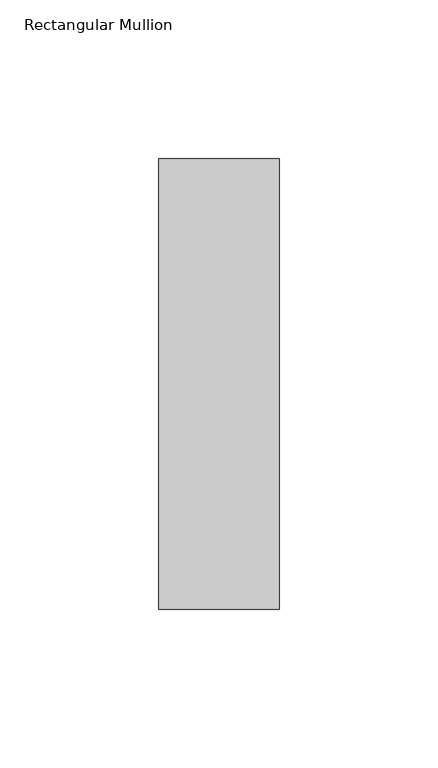
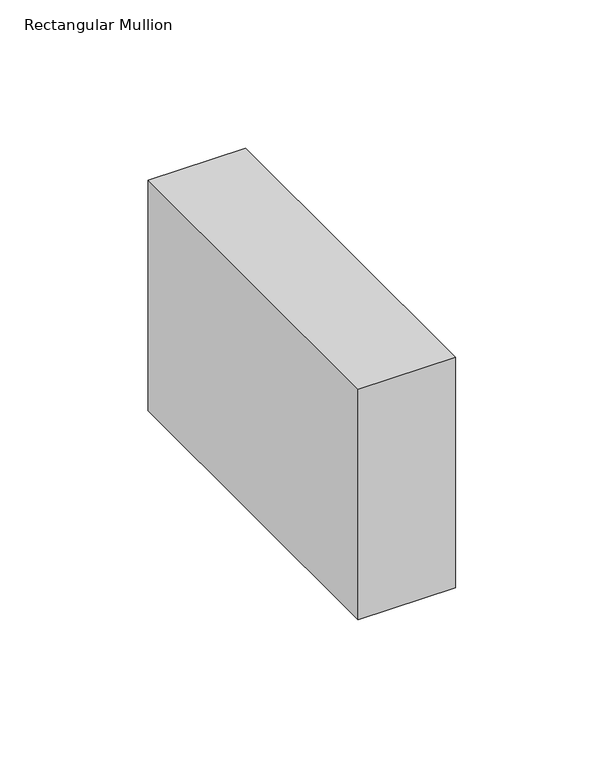
"""IFC4 building model written with IfcOpenShell, lengths in millimetres: member geometry, Rectangular Mullion : NLRS_21_CWM_hsb-regel 38x142_gen_rsf."""

from ifc_helpers import new_model, si_unit, frame, origin, place, context, project, spatial, polyline, outline, extrude, source, transform, mapped, element, save


def rectangular_mullion_3dbdc851(model_context):
    return source(origin(), model_context, "Body", "SweptSolid", [
        extrude(outline(polyline([(-38.0, -71.0), (-38.0, 71.0), (0.0, 71.0), (0.0, -71.0), (-38.0, -71.0)])), frame((0.0, 0.0, -94.9999997), z_axis=(0.0, 0.0, 1.0), x_axis=(1.0, 0.0, 0.0)), (0.0, 0.0, 1.0), 94.9999997),
    ])


if __name__ == "__main__":
    model = new_model("IFC4")
    model_context = context("Model", 3, world=origin())
    ifc_project = project(units=[si_unit("LENGTHUNIT", "METRE", prefix="MILLI")], contexts=[model_context])
    site = spatial("IfcSite", under=ifc_project)
    building = spatial("IfcBuilding", under=site)
    placement = place(None, origin())
    rectangular_mullion_shape = rectangular_mullion_3dbdc851(model_context)
    element("IfcMember", 1, ObjectType="Rectangular Mullion : NLRS_21_CWM_hsb-regel 38x142_gen_rsf", at=placement, inside=building, context=model_context, shape_type="MappedRepresentation", body=[
        mapped(rectangular_mullion_shape, transform((0.0, 0.0, 0.0), x_axis=(1.0, 0.0, 0.0), y_axis=(0.0, 1.0, 0.0), z_axis=(0.0, 0.0, 1.0))),
    ])
    save(model, "model.ifc")

# Revit data of these elements
# Type "Rectangular Mullion : NLRS_21_CWM_hsb-regel 38x142_gen_rsf"
#   Export Type to IFC As = "IfcWall"
#   Type IfcGUID = "07M7mRoiH1CR8m_RSKIwpF"
#   Assembly Code = "21.10"
#   built-in parameter 1007322 = 0.465879 (stored number, unit not read)
#   built-in parameter 1007321 = 0.062336 (stored number, unit not read)
#   built-in parameter 1007320 = 0.062336 (stored number, unit not read)
# Element 1 (IfcMember, "Rectangular Mullion : NLRS_21_CWM_hsb-regel 38x142_gen_rsf")
#   Materials on its faces: "NLRS_i2_hout naaldhout vuren_gen_rsf"
# Materials
#   "NLRS_i2_hout naaldhout vuren_gen_rsf": class "I - Hout", colour RGB 234 199 147, transparency 0, Keynote = "i2", Manufacturer = "Revit Standards Foundation", URL = "www.revitstandards.org", Description = "hout vuren", Cost = 0
